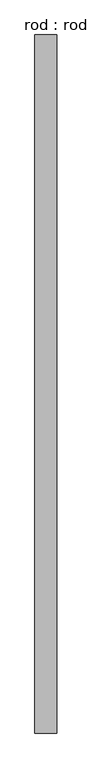
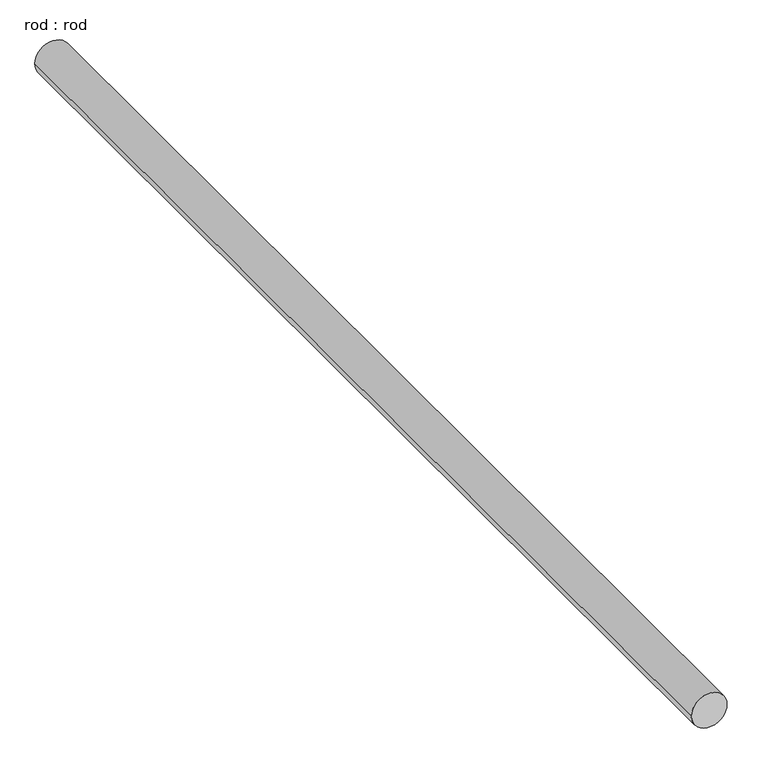
"""IFC4 building model written with IfcOpenShell, lengths in millimetres: proxy geometry, rod : rod."""

from ifc_helpers import new_model, si_unit, point, frame, frame_2d, origin, place, context, project, spatial, circle_curve, trimmed, segment, composite_curve, outline, extrude, source, transform, mapped, element, save


def rod_rod_ab447ccd(model_context):
    return source(origin(), model_context, "Body", "SweptSolid", [
        extrude(outline(composite_curve([segment(trimmed(circle_curve(frame_2d((0.0108462, 0.0)), 200.0), [point((0.0108462, 200.0))], [point((0.0108462, -200.0))], False, "CARTESIAN"), True, "CONTINUOUS"), segment(trimmed(circle_curve(frame_2d((0.0108462, 0.0)), 200.0), [point((0.0108462, -200.0))], [point((0.0108462, 200.0))], False, "CARTESIAN"), True, "CONTINUOUS")], self_intersect=False)), frame((0.0, -2268.4210611, 0.0), z_axis=(0.0, 1.0, 0.0), x_axis=(0.0, 0.0, 1.0)), (0.0, 0.0, 1.0), 12722.299353),
    ])


if __name__ == "__main__":
    model = new_model("IFC4")
    model_context = context("Model", 3, world=origin())
    ifc_project = project(units=[si_unit("LENGTHUNIT", "METRE", prefix="MILLI")], contexts=[model_context])
    site = spatial("IfcSite", under=ifc_project)
    building = spatial("IfcBuilding", under=site)
    placement = place(None, origin())
    rod_rod_shape = rod_rod_ab447ccd(model_context)
    element("IfcBuildingElementProxy", 1, Name="rod : rod", ObjectType="rod : rod", at=placement, inside=building, context=model_context, shape_type="MappedRepresentation", body=[
        mapped(rod_rod_shape, transform((0.0, 0.0, 0.0), x_axis=(1.0, 0.0, 0.0), y_axis=(0.0, 1.0, 0.0), z_axis=(0.0, 0.0, 1.0))),
    ])
    save(model, "model.ifc")

# Revit data of these elements
# Type "rod : rod"
#   Default Elevation = 0
